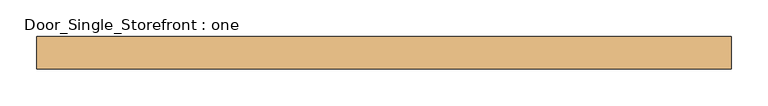
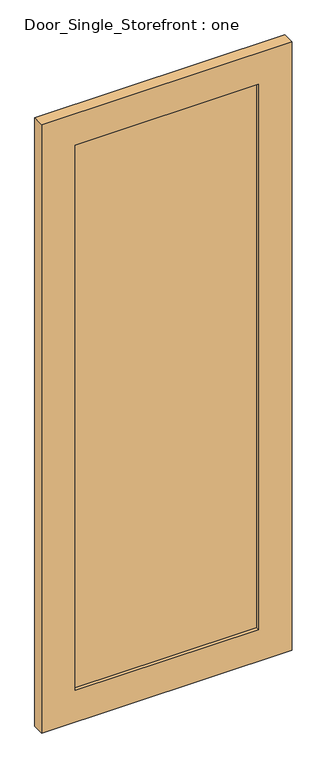
"""IFC4 building model written with IfcOpenShell, lengths in millimetres: door geometry, Door_Single_Storefront : one."""

from ifc_helpers import new_model, si_unit, frame, origin, place, context, project, spatial, polyline, outline, extrude, source, transform, mapped, element, save


def door_single_storefront_one_36bbcdfe(model_context):
    return source(origin(), model_context, "Body", "SweptSolid", [
        extrude(outline(polyline([(347.6625, -6.35), (-347.6625, -6.35), (-347.6625, 12.7), (347.6625, 12.7), (347.6625, -6.35)])), frame((0.0, 0.0, 127.0), z_axis=(0.0, 0.0, 1.0), x_axis=(1.0, 0.0, 0.0)), (0.0, 0.0, 1.0), 2184.4),
        extrude(outline(polyline([(2438.4, -474.6625), (0.0, -474.6625), (0.0, 474.6625), (2438.4, 474.6625), (2438.4, -474.6625)]), holes=[polyline([(127.0, 347.6625), (127.0, -347.6625), (2311.4, -347.6625), (2311.4, 347.6625), (127.0, 347.6625)])]), frame((0.0, -19.05, 0.0), z_axis=(0.0, 1.0, 0.0), x_axis=(0.0, 0.0, 1.0)), (0.0, 0.0, 1.0), 44.45),
    ])


if __name__ == "__main__":
    model = new_model("IFC4")
    model_context = context("Model", 3, world=origin())
    ifc_project = project(units=[si_unit("LENGTHUNIT", "METRE", prefix="MILLI")], contexts=[model_context])
    site = spatial("IfcSite", under=ifc_project)
    building = spatial("IfcBuilding", under=site)
    placement = place(None, origin())
    door_single_storefront_one_shape = door_single_storefront_one_36bbcdfe(model_context)
    element("IfcDoor", 1, ObjectType="Door_Single_Storefront : one", at=placement, inside=building, context=model_context, shape_type="MappedRepresentation", body=[
        mapped(door_single_storefront_one_shape, transform((0.0, 0.0, 0.0), x_axis=(1.0, 0.0, 0.0), y_axis=(0.0, 1.0, 0.0), z_axis=(0.0, 0.0, 1.0))),
    ])
    save(model, "model.ifc")

# Revit data of these elements
# Type "Door_Single_Storefront : one"
#   Type Mark = "27"
#   Analytic Construction = "<None>"
#   Stile_Width = 0' - 5"
#   Door_Thickness = 0' - 1 3/4"
#   Door_Offset = 0' - 1"
#   Glass_Material = SAFETY GLAZING
#   Frame_Material = INTERIOR GRADE ALUMINUM STOREFRONT W/ SAFETY GLAZING
#   Function = (empty or 0)
# Element 1 (IfcDoor, "Door_Single_Storefront : one")
#   Materials on its faces: "INTERIOR GRADE ALUMINUM STOREFRONT W/ SAFETY GLAZING", "SAFETY GLAZING"
# Materials
#   "SAFETY GLAZING": class "Glass", colour RGB 142 168 196, transparency 0.75, Description = "Soda Lime Glass", Cost = 0
#   "INTERIOR GRADE ALUMINUM STOREFRONT W/ SAFETY GLAZING": class "Metal", colour RGB 226 226 226, transparency 0, Description = "Aluminum 6061", Cost = 0
